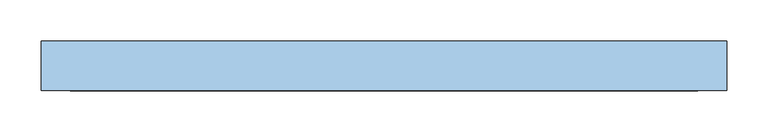
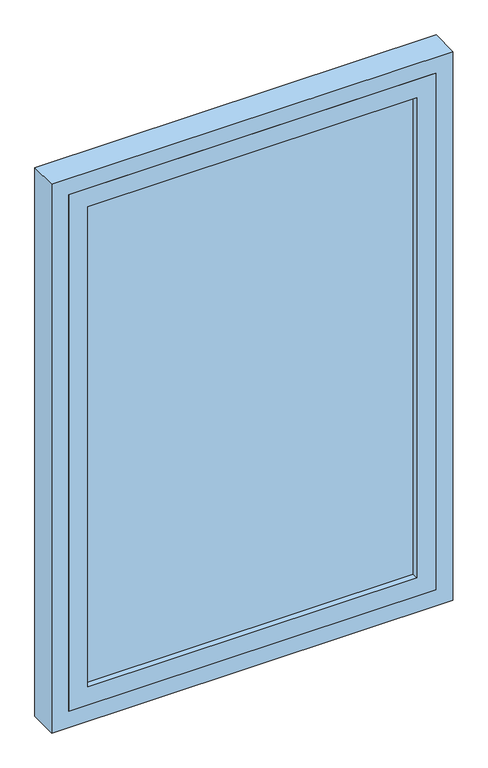
"""IFC4 building model written with IfcOpenShell, lengths in millimetres: window geometry, Janela fixa - 1 Painel : Janela fixa - 1 Painel."""

import ifcopenshell
import ifcopenshell.guid

model = None  # the IFC model being written
_history = None  # IfcOwnerHistory: only IFC2X3 demands one
_inside = {}  # id of a spatial element -> (the spatial element, [elements in it])
_under = {}  # id of a project, library or spatial element -> (it, [spatial elements below it])
_declared = {}  # id of a project -> (the project, [libraries it declares])
_typed = {}  # id of a type object -> (the type object, [elements of that type])
_made_of = {}  # id of a material, layer set ... -> (it, [elements and type objects made of it])


def new_model(schema):
    """Start an empty IFC model of exactly this schema.

    Asked for "IFC4X3", IfcOpenShell would pick the latest addendum, in which some entities
    have other attributes; the version numbers below select the first issue.
    IFC2X3 requires an IfcOwnerHistory on every rooted entity: one is made here for all.
    """
    global model, _history
    if schema == "IFC4X3":
        model = ifcopenshell.file(schema_version=(4, 3, 0, 0))
    else:
        model = ifcopenshell.file(schema=schema)
    _inside.clear()
    _under.clear()
    _declared.clear()
    _typed.clear()
    _made_of.clear()
    _history = None
    if model.schema == "IFC2X3":
        org = make("IfcOrganization", Name="unknown")
        user = make(
            "IfcPersonAndOrganization",
            ThePerson=make("IfcPerson", FamilyName="unknown"),
            TheOrganization=org,
        )
        app = make(
            "IfcApplication",
            ApplicationDeveloper=org,
            Version="unknown",
            ApplicationFullName="unknown",
            ApplicationIdentifier="unknown",
        )
        _history = make(
            "IfcOwnerHistory",
            OwningUser=user,
            OwningApplication=app,
            ChangeAction="ADDED",
            CreationDate=0,
        )
    return model


def make(cls, **values):
    """One entity of the class cls with the attributes given. An attribute that is None is left unset."""
    return model.create_entity(
        cls, **{name: value for name, value in values.items() if value is not None}
    )


def rooted(cls, **values):
    """An entity with a GlobalId (a new one), such as an element, a storey or a relation."""
    return make(cls, GlobalId=ifcopenshell.guid.new(), OwnerHistory=_history, **values)


def si_unit(unit_type, name, prefix=None):
    """IfcSIUnit, for example si_unit("LENGTHUNIT", "METRE", prefix="MILLI")."""
    return make("IfcSIUnit", UnitType=unit_type, Prefix=prefix, Name=name)


def assignment(units):
    """IfcUnitAssignment: the units of a project."""
    return None if units is None else make("IfcUnitAssignment", Units=units)


def point(xyz):
    """IfcCartesianPoint."""
    return None if xyz is None else make("IfcCartesianPoint", Coordinates=xyz)


def direction(xyz):
    """IfcDirection."""
    return None if xyz is None else make("IfcDirection", DirectionRatios=xyz)


def frame(location, z_axis=None, x_axis=None):
    """IfcAxis2Placement3D, a coordinate frame: its origin and axes. An axis left out is left unset."""
    return make(
        "IfcAxis2Placement3D",
        Location=point(location),
        Axis=direction(z_axis),
        RefDirection=direction(x_axis),
    )


def origin():
    """The frame at (0, 0, 0) with its axes left unset."""
    return frame((0.0, 0.0, 0.0))


def place(relative_to, where):
    """IfcLocalPlacement: puts the frame where relative to a parent placement (None: the world)."""
    return make(
        "IfcLocalPlacement", PlacementRelTo=relative_to, RelativePlacement=where
    )


def context(
    kind, dimensions, precision=None, world=None, true_north=None, identifier=None
):
    """IfcGeometricRepresentationContext, for example the 3D "Model" context."""
    return make(
        "IfcGeometricRepresentationContext",
        ContextIdentifier=identifier,
        ContextType=kind,
        CoordinateSpaceDimension=dimensions,
        Precision=precision,
        WorldCoordinateSystem=world,
        TrueNorth=true_north,
    )


def project(units=None, contexts=None):
    """IfcProject with its units and contexts."""
    return rooted(
        "IfcProject",
        Name="project",
        RepresentationContexts=contexts,
        UnitsInContext=assignment(units),
    )


def spatial(cls, under=None, at=None, **own):
    """A site, building, storey or space (cls), placed at a placement, below another one or the project."""
    s = rooted(cls, ObjectPlacement=at, **own)
    if under is not None:
        _under.setdefault(under.id(), (under, []))[1].append(s)
    return s


def polyline(points):
    """IfcPolyline through the points."""
    return make("IfcPolyline", Points=[point(p) for p in points])


def outline(outer, holes=None, kind="AREA"):
    """IfcArbitraryClosedProfileDef: a profile drawn as a closed curve; with holes, ...WithVoids."""
    if holes is None:
        return make("IfcArbitraryClosedProfileDef", ProfileType=kind, OuterCurve=outer)
    return make(
        "IfcArbitraryProfileDefWithVoids",
        ProfileType=kind,
        OuterCurve=outer,
        InnerCurves=holes,
    )


def extrude(swept, where, along, depth):
    """IfcExtrudedAreaSolid: the profile swept, set in the frame where, extruded along a direction by depth."""
    return make(
        "IfcExtrudedAreaSolid",
        SweptArea=swept,
        Position=where,
        ExtrudedDirection=direction(along),
        Depth=depth,
    )


def shape(context_of_items, identifier, shape_type, items):
    """IfcShapeRepresentation: the items that make up one representation, for example the "Body"."""
    return make(
        "IfcShapeRepresentation",
        ContextOfItems=context_of_items,
        RepresentationIdentifier=identifier,
        RepresentationType=shape_type,
        Items=items,
    )


def source(mapping_origin, context_of_items, identifier, shape_type, items):
    """IfcRepresentationMap: a shape defined once, which mapped items show again and again."""
    return make(
        "IfcRepresentationMap",
        MappingOrigin=mapping_origin,
        MappedRepresentation=shape(context_of_items, identifier, shape_type, items),
    )


def transform(
    local_origin,
    x_axis=None,
    y_axis=None,
    z_axis=None,
    scale=None,
    scale2=None,
    scale3=None,
    uniform=True,
):
    """IfcCartesianTransformationOperator3D, or its non-uniform kind. x_axis, y_axis, z_axis: its Axis1, 2, 3."""
    if uniform:
        return make(
            "IfcCartesianTransformationOperator3D",
            Axis1=direction(x_axis),
            Axis2=direction(y_axis),
            LocalOrigin=point(local_origin),
            Scale=scale,
            Axis3=direction(z_axis),
        )
    return make(
        "IfcCartesianTransformationOperator3DnonUniform",
        Axis1=direction(x_axis),
        Axis2=direction(y_axis),
        LocalOrigin=point(local_origin),
        Scale=scale,
        Axis3=direction(z_axis),
        Scale2=scale2,
        Scale3=scale3,
    )


def mapped(mapping_source, mapping_target):
    """IfcMappedItem: shows the shape of a source again, moved by a transform."""
    return make(
        "IfcMappedItem", MappingSource=mapping_source, MappingTarget=mapping_target
    )


def made_of(thing, what):
    """Note that an element or type object is made of a material, layer set ...; save() writes the relation."""
    if what is not None:
        _made_of.setdefault(what.id(), (what, []))[1].append(thing)
    return thing


def element(
    cls,
    number,
    at=None,
    inside=None,
    cuts=None,
    type_object=None,
    material=None,
    context=None,
    identifier="Body",
    shape_type=None,
    held_by="IfcProductDefinitionShape",
    body=None,
    shapes=None,
    **own,
):
    """One element of the class cls, such as IfcWall. Its Tag is "e" and its number.

    at: its placement. inside: the storey or other place that contains it. cuts: it is an
    opening in that element (IfcRelVoidsElement). A single representation is given by context,
    identifier, shape_type and body (its items); several are given by shapes. held_by: the class
    of the entity that holds the representations. save() writes the other relations.
    """
    e = rooted(cls, Tag="e%d" % number, ObjectPlacement=at, **own)
    if body is not None:
        shapes = [shape(context, identifier, shape_type, body)]
    if shapes is not None:
        e.Representation = make(held_by, Representations=shapes)
    if inside is not None:
        _inside.setdefault(inside.id(), (inside, []))[1].append(e)
    if cuts is not None:
        rooted(
            "IfcRelVoidsElement", RelatingBuildingElement=cuts, RelatedOpeningElement=e
        )
    if type_object is not None:
        _typed.setdefault(type_object.id(), (type_object, []))[1].append(e)
    return made_of(e, material)


def aggregate(whole, parts):
    """IfcRelAggregates: a whole, such as a stair, and the parts it consists of."""
    return rooted("IfcRelAggregates", RelatingObject=whole, RelatedObjects=parts)


def save(model, path):
    """Write the relations noted so far, then the file.

    IfcRelAggregates (storeys below a building ...), IfcRelContainedInSpatialStructure (elements
    in a storey), IfcRelDefinesByType, IfcRelAssociatesMaterial and IfcRelDeclares: one each for
    every whole, place, type object, material and project.
    """
    for whole, parts in _under.values():
        aggregate(whole, parts)
    for where, things in _inside.values():
        rooted(
            "IfcRelContainedInSpatialStructure",
            RelatedElements=things,
            RelatingStructure=where,
        )
    for kind, things in _typed.values():
        rooted("IfcRelDefinesByType", RelatedObjects=things, RelatingType=kind)
    for what, things in _made_of.values():
        rooted("IfcRelAssociatesMaterial", RelatedObjects=things, RelatingMaterial=what)
    for by, libraries in _declared.values():
        rooted("IfcRelDeclares", RelatingContext=by, RelatedDefinitions=libraries)
    model.write(path)


def window_71ad020b(model_context):
    return source(origin(), model_context, "Body", "SweptSolid", [
        extrude(outline(polyline([(340.0, -52.6), (340.0, -66.6), (-340.0, -66.6), (-340.0, -52.6), (340.0, -52.6)])), frame((0.0, 0.0, 725.0), z_axis=(0.0, 0.0, 1.0), x_axis=(1.0, 0.0, 0.0)), (0.0, 0.0, 1.0), 1050.0),
        extrude(outline(polyline([(685.0, -380.0), (685.0, 380.0), (1815.0, 380.0), (1815.0, -380.0), (685.0, -380.0)]), holes=[polyline([(1775.0, -340.0), (1775.0, 340.0), (725.0, 340.0), (725.0, -340.0), (1775.0, -340.0)])]), frame((0.0, -79.6, 0.0), z_axis=(0.0, 1.0, 0.0), x_axis=(0.0, 0.0, 1.0)), (0.0, 0.0, 1.0), 40.0),
        extrude(outline(polyline([(650.0, -415.0), (650.0, 415.0), (1850.0, 415.0), (1850.0, -415.0), (650.0, -415.0)]), holes=[polyline([(1815.0, -380.0), (1815.0, 380.0), (685.0, 380.0), (685.0, -380.0), (1815.0, -380.0)])]), frame((0.0, -79.6, 0.0), z_axis=(0.0, 1.0, 0.0), x_axis=(0.0, 0.0, 1.0)), (0.0, 0.0, 1.0), 60.0),
    ])


if __name__ == "__main__":
    model = new_model("IFC4")
    model_context = context("Model", 3, world=origin())
    ifc_project = project(units=[si_unit("LENGTHUNIT", "METRE", prefix="MILLI")], contexts=[model_context])
    site = spatial("IfcSite", under=ifc_project)
    building = spatial("IfcBuilding", under=site)
    placement = place(None, origin())
    window_shape = window_71ad020b(model_context)
    element("IfcWindow", 1, ObjectType="Janela fixa - 1 Painel : Janela fixa - 1 Painel", at=placement, inside=building, context=model_context, shape_type="MappedRepresentation", body=[
        mapped(window_shape, transform((0.0, 0.0, 0.0), x_axis=(1.0, 0.0, 0.0), y_axis=(0.0, 1.0, 0.0), z_axis=(0.0, 0.0, 1.0))),
    ])
    save(model, "model.ifc")

# Revit data of these elements
# Type "Janela fixa - 1 Painel : Janela fixa - 1 Painel"
#   Type Mark = "J15"
#   Construction Type Id = "SGL"
#   Analytic Construction = "Janelas grandes envidraçadas únicas"
#   Visual Light Transmittance = 0.9
#   Solar Heat Gain Coefficient = 0.86
#   Rough Width = 0.83 m
#   Rough Height = 1.20 m
#   Largura da moldura do painel = 0.04 m
#   Espessura da moldura do painel = 0.04 m
#   Height = 1.20 m
#   Heat Transfer Coefficient (U) = 5.5617 W/(m²·K)
#   Largura da estrutura = 0.035 m
#   Espessura da moldura = 0.06 m
#   Altura-padrão do peitoril = 0.65 m
#   Width = 0.83 m
#   Vidro = Vidro - Janela
#   Material da estrutura = Aluminum Sill
#   Wall Closure = (empty or 0)
# Element 1 (IfcWindow, "Janela fixa - 1 Painel : Janela fixa - 1 Painel")
#   Materials on its faces: "Aluminum Sill", "Vidro - Janela"
# Materials
#   "Vidro - Janela": class "Vidro", colour RGB 249 249 249, transparency 1, Cost = 0
#   "Aluminum Sill": class "Não atribuído", colour RGB 247 247 247, transparency 0
